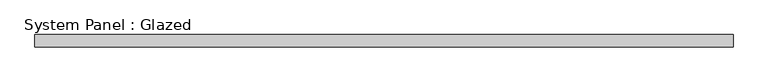
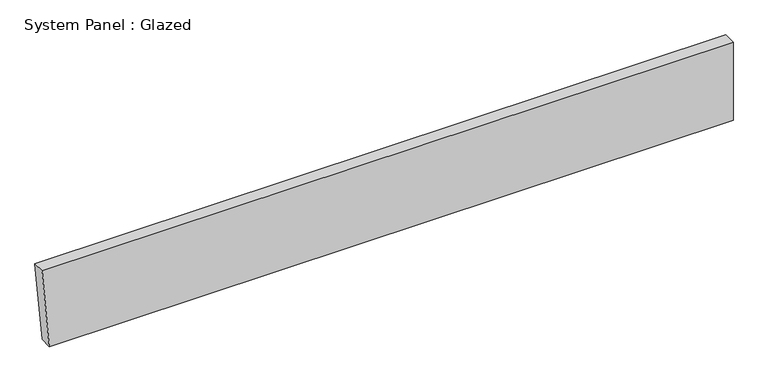
"""IFC4 building model written with IfcOpenShell, lengths in millimetres: plate geometry, System Panel : Glazed."""

import ifcopenshell
import ifcopenshell.guid

model = None  # the IFC model being written
_history = None  # IfcOwnerHistory: only IFC2X3 demands one
_inside = {}  # id of a spatial element -> (the spatial element, [elements in it])
_under = {}  # id of a project, library or spatial element -> (it, [spatial elements below it])
_declared = {}  # id of a project -> (the project, [libraries it declares])
_typed = {}  # id of a type object -> (the type object, [elements of that type])
_made_of = {}  # id of a material, layer set ... -> (it, [elements and type objects made of it])


def new_model(schema):
    """Start an empty IFC model of exactly this schema.

    Asked for "IFC4X3", IfcOpenShell would pick the latest addendum, in which some entities
    have other attributes; the version numbers below select the first issue.
    IFC2X3 requires an IfcOwnerHistory on every rooted entity: one is made here for all.
    """
    global model, _history
    if schema == "IFC4X3":
        model = ifcopenshell.file(schema_version=(4, 3, 0, 0))
    else:
        model = ifcopenshell.file(schema=schema)
    _inside.clear()
    _under.clear()
    _declared.clear()
    _typed.clear()
    _made_of.clear()
    _history = None
    if model.schema == "IFC2X3":
        org = make("IfcOrganization", Name="unknown")
        user = make(
            "IfcPersonAndOrganization",
            ThePerson=make("IfcPerson", FamilyName="unknown"),
            TheOrganization=org,
        )
        app = make(
            "IfcApplication",
            ApplicationDeveloper=org,
            Version="unknown",
            ApplicationFullName="unknown",
            ApplicationIdentifier="unknown",
        )
        _history = make(
            "IfcOwnerHistory",
            OwningUser=user,
            OwningApplication=app,
            ChangeAction="ADDED",
            CreationDate=0,
        )
    return model


def make(cls, **values):
    """One entity of the class cls with the attributes given. An attribute that is None is left unset."""
    return model.create_entity(
        cls, **{name: value for name, value in values.items() if value is not None}
    )


def rooted(cls, **values):
    """An entity with a GlobalId (a new one), such as an element, a storey or a relation."""
    return make(cls, GlobalId=ifcopenshell.guid.new(), OwnerHistory=_history, **values)


def si_unit(unit_type, name, prefix=None):
    """IfcSIUnit, for example si_unit("LENGTHUNIT", "METRE", prefix="MILLI")."""
    return make("IfcSIUnit", UnitType=unit_type, Prefix=prefix, Name=name)


def assignment(units):
    """IfcUnitAssignment: the units of a project."""
    return None if units is None else make("IfcUnitAssignment", Units=units)


def point(xyz):
    """IfcCartesianPoint."""
    return None if xyz is None else make("IfcCartesianPoint", Coordinates=xyz)


def direction(xyz):
    """IfcDirection."""
    return None if xyz is None else make("IfcDirection", DirectionRatios=xyz)


def frame(location, z_axis=None, x_axis=None):
    """IfcAxis2Placement3D, a coordinate frame: its origin and axes. An axis left out is left unset."""
    return make(
        "IfcAxis2Placement3D",
        Location=point(location),
        Axis=direction(z_axis),
        RefDirection=direction(x_axis),
    )


def origin():
    """The frame at (0, 0, 0) with its axes left unset."""
    return frame((0.0, 0.0, 0.0))


def place(relative_to, where):
    """IfcLocalPlacement: puts the frame where relative to a parent placement (None: the world)."""
    return make(
        "IfcLocalPlacement", PlacementRelTo=relative_to, RelativePlacement=where
    )


def context(
    kind, dimensions, precision=None, world=None, true_north=None, identifier=None
):
    """IfcGeometricRepresentationContext, for example the 3D "Model" context."""
    return make(
        "IfcGeometricRepresentationContext",
        ContextIdentifier=identifier,
        ContextType=kind,
        CoordinateSpaceDimension=dimensions,
        Precision=precision,
        WorldCoordinateSystem=world,
        TrueNorth=true_north,
    )


def project(units=None, contexts=None):
    """IfcProject with its units and contexts."""
    return rooted(
        "IfcProject",
        Name="project",
        RepresentationContexts=contexts,
        UnitsInContext=assignment(units),
    )


def spatial(cls, under=None, at=None, **own):
    """A site, building, storey or space (cls), placed at a placement, below another one or the project."""
    s = rooted(cls, ObjectPlacement=at, **own)
    if under is not None:
        _under.setdefault(under.id(), (under, []))[1].append(s)
    return s


def polyline(points):
    """IfcPolyline through the points."""
    return make("IfcPolyline", Points=[point(p) for p in points])


def outline(outer, holes=None, kind="AREA"):
    """IfcArbitraryClosedProfileDef: a profile drawn as a closed curve; with holes, ...WithVoids."""
    if holes is None:
        return make("IfcArbitraryClosedProfileDef", ProfileType=kind, OuterCurve=outer)
    return make(
        "IfcArbitraryProfileDefWithVoids",
        ProfileType=kind,
        OuterCurve=outer,
        InnerCurves=holes,
    )


def extrude(swept, where, along, depth):
    """IfcExtrudedAreaSolid: the profile swept, set in the frame where, extruded along a direction by depth."""
    return make(
        "IfcExtrudedAreaSolid",
        SweptArea=swept,
        Position=where,
        ExtrudedDirection=direction(along),
        Depth=depth,
    )


def shape(context_of_items, identifier, shape_type, items):
    """IfcShapeRepresentation: the items that make up one representation, for example the "Body"."""
    return make(
        "IfcShapeRepresentation",
        ContextOfItems=context_of_items,
        RepresentationIdentifier=identifier,
        RepresentationType=shape_type,
        Items=items,
    )


def source(mapping_origin, context_of_items, identifier, shape_type, items):
    """IfcRepresentationMap: a shape defined once, which mapped items show again and again."""
    return make(
        "IfcRepresentationMap",
        MappingOrigin=mapping_origin,
        MappedRepresentation=shape(context_of_items, identifier, shape_type, items),
    )


def transform(
    local_origin,
    x_axis=None,
    y_axis=None,
    z_axis=None,
    scale=None,
    scale2=None,
    scale3=None,
    uniform=True,
):
    """IfcCartesianTransformationOperator3D, or its non-uniform kind. x_axis, y_axis, z_axis: its Axis1, 2, 3."""
    if uniform:
        return make(
            "IfcCartesianTransformationOperator3D",
            Axis1=direction(x_axis),
            Axis2=direction(y_axis),
            LocalOrigin=point(local_origin),
            Scale=scale,
            Axis3=direction(z_axis),
        )
    return make(
        "IfcCartesianTransformationOperator3DnonUniform",
        Axis1=direction(x_axis),
        Axis2=direction(y_axis),
        LocalOrigin=point(local_origin),
        Scale=scale,
        Axis3=direction(z_axis),
        Scale2=scale2,
        Scale3=scale3,
    )


def mapped(mapping_source, mapping_target):
    """IfcMappedItem: shows the shape of a source again, moved by a transform."""
    return make(
        "IfcMappedItem", MappingSource=mapping_source, MappingTarget=mapping_target
    )


def made_of(thing, what):
    """Note that an element or type object is made of a material, layer set ...; save() writes the relation."""
    if what is not None:
        _made_of.setdefault(what.id(), (what, []))[1].append(thing)
    return thing


def element(
    cls,
    number,
    at=None,
    inside=None,
    cuts=None,
    type_object=None,
    material=None,
    context=None,
    identifier="Body",
    shape_type=None,
    held_by="IfcProductDefinitionShape",
    body=None,
    shapes=None,
    **own,
):
    """One element of the class cls, such as IfcWall. Its Tag is "e" and its number.

    at: its placement. inside: the storey or other place that contains it. cuts: it is an
    opening in that element (IfcRelVoidsElement). A single representation is given by context,
    identifier, shape_type and body (its items); several are given by shapes. held_by: the class
    of the entity that holds the representations. save() writes the other relations.
    """
    e = rooted(cls, Tag="e%d" % number, ObjectPlacement=at, **own)
    if body is not None:
        shapes = [shape(context, identifier, shape_type, body)]
    if shapes is not None:
        e.Representation = make(held_by, Representations=shapes)
    if inside is not None:
        _inside.setdefault(inside.id(), (inside, []))[1].append(e)
    if cuts is not None:
        rooted(
            "IfcRelVoidsElement", RelatingBuildingElement=cuts, RelatedOpeningElement=e
        )
    if type_object is not None:
        _typed.setdefault(type_object.id(), (type_object, []))[1].append(e)
    return made_of(e, material)


def aggregate(whole, parts):
    """IfcRelAggregates: a whole, such as a stair, and the parts it consists of."""
    return rooted("IfcRelAggregates", RelatingObject=whole, RelatedObjects=parts)


def save(model, path):
    """Write the relations noted so far, then the file.

    IfcRelAggregates (storeys below a building ...), IfcRelContainedInSpatialStructure (elements
    in a storey), IfcRelDefinesByType, IfcRelAssociatesMaterial and IfcRelDeclares: one each for
    every whole, place, type object, material and project.
    """
    for whole, parts in _under.values():
        aggregate(whole, parts)
    for where, things in _inside.values():
        rooted(
            "IfcRelContainedInSpatialStructure",
            RelatedElements=things,
            RelatingStructure=where,
        )
    for kind, things in _typed.values():
        rooted("IfcRelDefinesByType", RelatedObjects=things, RelatingType=kind)
    for what, things in _made_of.values():
        rooted("IfcRelAssociatesMaterial", RelatedObjects=things, RelatingMaterial=what)
    for by, libraries in _declared.values():
        rooted("IfcRelDeclares", RelatingContext=by, RelatedDefinitions=libraries)
    model.write(path)


def system_panel_glazed_d86b06c2(model_context):
    return source(origin(), model_context, "Body", "SweptSolid", [
        extrude(outline(polyline([(0.0, -694.0133132), (0.0, 708.5978036), (169.2731269, 708.5978036), (169.2731269, -708.5978036), (0.0, -694.0133132)])), frame((0.0, -44.45, 0.0), z_axis=(0.0, 1.0, 0.0), x_axis=(0.0, 0.0, 1.0)), (0.0, 0.0, 1.0), 25.4),
    ])


if __name__ == "__main__":
    model = new_model("IFC4")
    model_context = context("Model", 3, world=origin())
    ifc_project = project(units=[si_unit("LENGTHUNIT", "METRE", prefix="MILLI")], contexts=[model_context])
    site = spatial("IfcSite", under=ifc_project)
    building = spatial("IfcBuilding", under=site)
    placement = place(None, origin())
    system_panel_glazed_shape = system_panel_glazed_d86b06c2(model_context)
    element("IfcPlate", 1, ObjectType="System Panel : Glazed", at=placement, inside=building, context=model_context, shape_type="MappedRepresentation", body=[
        mapped(system_panel_glazed_shape, transform((0.0, 0.0, 0.0), x_axis=(1.0, 0.0, 0.0), y_axis=(0.0, 1.0, 0.0), z_axis=(0.0, 0.0, 1.0))),
    ])
    save(model, "model.ifc")

# Revit data of these elements
# Type "System Panel : Glazed"
#   Construction Type Id = "GSP4R"
#   Analytic Construction = "1/8 in Pilkington single glazing"
#   Visual Light Transmittance = 0.9
#   Solar Heat Gain Coefficient = 0.86
#   Heat Transfer Coefficient (U) = 1.18115 BTU/(h·ft²·°F)
#   Define Thermal Properties by = 1
# Element 1 (IfcPlate, "System Panel : Glazed")
#   Materials on its faces: "Glass"
# Materials
#   "Glass": class "Glass", colour RGB 0 128 192, transparency 0.75, Description = "Soda Lime Glass", Cost = 0
